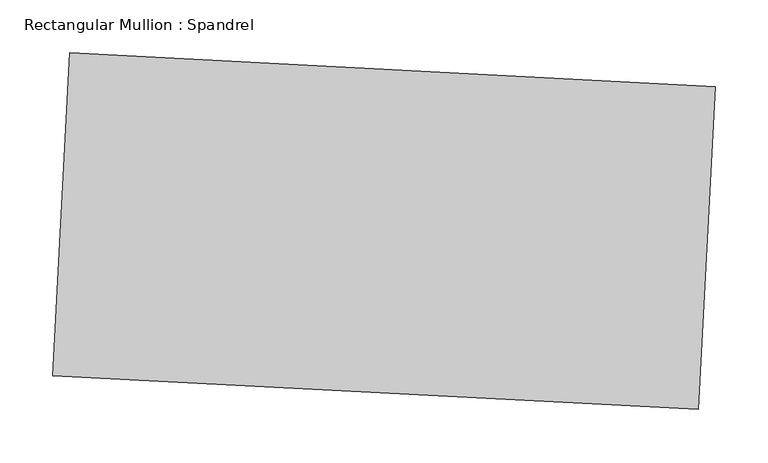
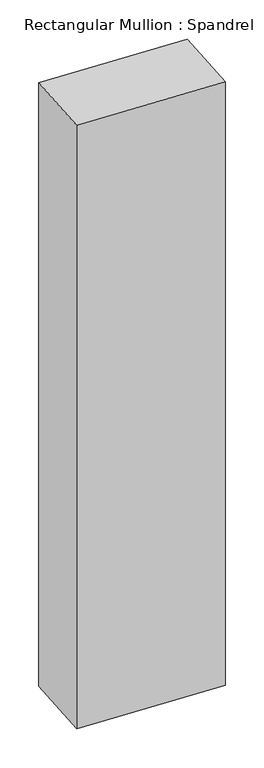
"""IFC4 building model written with IfcOpenShell, lengths in millimetres: member geometry, Rectangular Mullion : Spandrel."""

from ifc_helpers import new_model, si_unit, frame, origin, place, context, project, spatial, polyline, outline, extrude, source, transform, mapped, element, save


def rectangular_mullion_spandrel_57f4b63b(model_context):
    return source(origin(), model_context, "Body", "SweptSolid", [
        extrude(outline(polyline([(312.3582819, 136.2391416), (296.4062825, -168.1431406), (-312.3582819, -136.2391416), (-296.4062825, 168.1431406), (312.3582819, 136.2391416)])), frame((0.0, 0.0, -2693.0670444), z_axis=(0.0, 0.0, 1.0), x_axis=(1.0, 0.0, 0.0)), (0.0, 0.0, 1.0), 2693.0670444),
    ])


if __name__ == "__main__":
    model = new_model("IFC4")
    model_context = context("Model", 3, world=origin())
    ifc_project = project(units=[si_unit("LENGTHUNIT", "METRE", prefix="MILLI")], contexts=[model_context])
    site = spatial("IfcSite", under=ifc_project)
    building = spatial("IfcBuilding", under=site)
    placement = place(None, origin())
    rectangular_mullion_spandrel_shape = rectangular_mullion_spandrel_57f4b63b(model_context)
    element("IfcMember", 1, ObjectType="Rectangular Mullion : Spandrel", at=placement, inside=building, context=model_context, shape_type="MappedRepresentation", body=[
        mapped(rectangular_mullion_spandrel_shape, transform((0.0, 0.0, 0.0), x_axis=(1.0, 0.0, 0.0), y_axis=(0.0, 1.0, 0.0), z_axis=(0.0, 0.0, 1.0))),
    ])
    save(model, "model.ifc")

# Revit data of these elements
# Type "Rectangular Mullion : Spandrel"
#   built-in parameter 1007304 = 1 (stored number, unit not read)
#   built-in parameter 1007301 = 1 (stored number, unit not read)
#   built-in parameter 1007300 = 1 (stored number, unit not read)
# Element 1 (IfcMember, "Rectangular Mullion : Spandrel")
#   Materials on its faces: "Aluminum"
# Materials
#   "Aluminum": class "Metal", colour RGB 247 247 247, transparency 0, Description = "Aluminum 6061", Cost = 0
